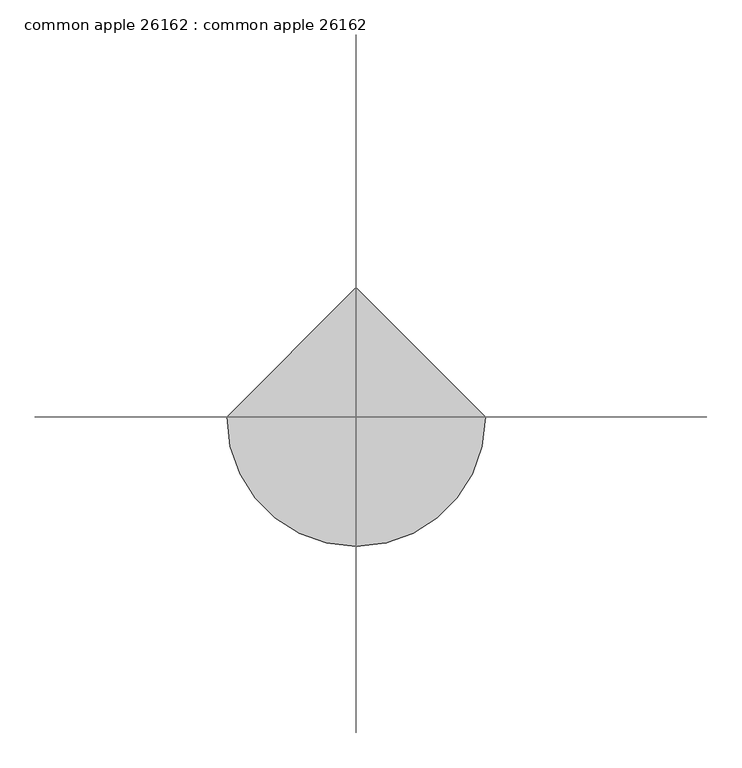
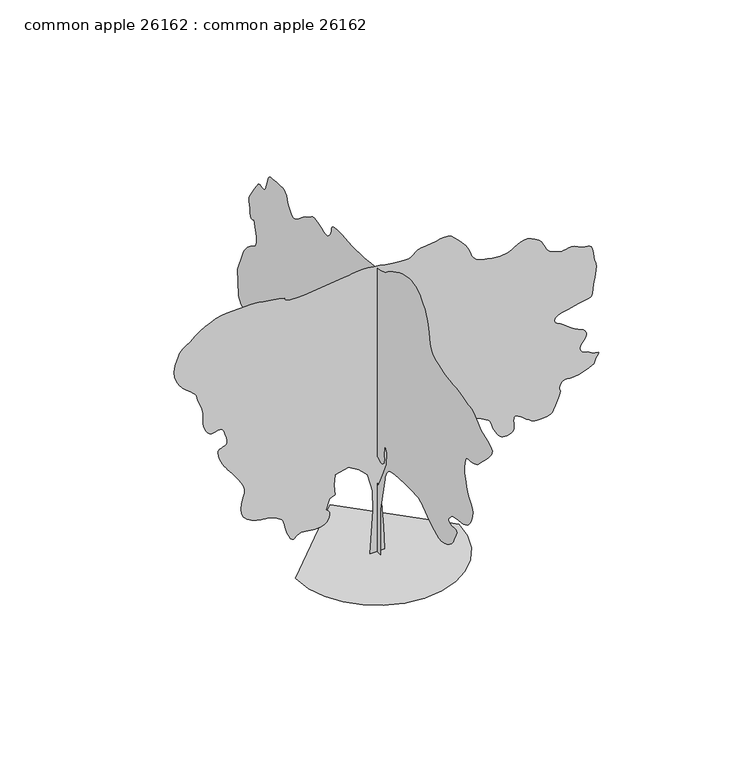
"""IFC4 building model written with IfcOpenShell, lengths in millimetres: proxy geometry, common apple 26162 : common apple 26162."""

import ifcopenshell
import ifcopenshell.guid

model = None  # the IFC model being written
_history = None  # IfcOwnerHistory: only IFC2X3 demands one
_inside = {}  # id of a spatial element -> (the spatial element, [elements in it])
_under = {}  # id of a project, library or spatial element -> (it, [spatial elements below it])
_declared = {}  # id of a project -> (the project, [libraries it declares])
_typed = {}  # id of a type object -> (the type object, [elements of that type])
_made_of = {}  # id of a material, layer set ... -> (it, [elements and type objects made of it])


def new_model(schema):
    """Start an empty IFC model of exactly this schema.

    Asked for "IFC4X3", IfcOpenShell would pick the latest addendum, in which some entities
    have other attributes; the version numbers below select the first issue.
    IFC2X3 requires an IfcOwnerHistory on every rooted entity: one is made here for all.
    """
    global model, _history
    if schema == "IFC4X3":
        model = ifcopenshell.file(schema_version=(4, 3, 0, 0))
    else:
        model = ifcopenshell.file(schema=schema)
    _inside.clear()
    _under.clear()
    _declared.clear()
    _typed.clear()
    _made_of.clear()
    _history = None
    if model.schema == "IFC2X3":
        org = make("IfcOrganization", Name="unknown")
        user = make(
            "IfcPersonAndOrganization",
            ThePerson=make("IfcPerson", FamilyName="unknown"),
            TheOrganization=org,
        )
        app = make(
            "IfcApplication",
            ApplicationDeveloper=org,
            Version="unknown",
            ApplicationFullName="unknown",
            ApplicationIdentifier="unknown",
        )
        _history = make(
            "IfcOwnerHistory",
            OwningUser=user,
            OwningApplication=app,
            ChangeAction="ADDED",
            CreationDate=0,
        )
    return model


def make(cls, **values):
    """One entity of the class cls with the attributes given. An attribute that is None is left unset."""
    return model.create_entity(
        cls, **{name: value for name, value in values.items() if value is not None}
    )


def rooted(cls, **values):
    """An entity with a GlobalId (a new one), such as an element, a storey or a relation."""
    return make(cls, GlobalId=ifcopenshell.guid.new(), OwnerHistory=_history, **values)


def si_unit(unit_type, name, prefix=None):
    """IfcSIUnit, for example si_unit("LENGTHUNIT", "METRE", prefix="MILLI")."""
    return make("IfcSIUnit", UnitType=unit_type, Prefix=prefix, Name=name)


def assignment(units):
    """IfcUnitAssignment: the units of a project."""
    return None if units is None else make("IfcUnitAssignment", Units=units)


def point(xyz):
    """IfcCartesianPoint."""
    return None if xyz is None else make("IfcCartesianPoint", Coordinates=xyz)


def direction(xyz):
    """IfcDirection."""
    return None if xyz is None else make("IfcDirection", DirectionRatios=xyz)


def frame(location, z_axis=None, x_axis=None):
    """IfcAxis2Placement3D, a coordinate frame: its origin and axes. An axis left out is left unset."""
    return make(
        "IfcAxis2Placement3D",
        Location=point(location),
        Axis=direction(z_axis),
        RefDirection=direction(x_axis),
    )


def origin():
    """The frame at (0, 0, 0) with its axes left unset."""
    return frame((0.0, 0.0, 0.0))


def place(relative_to, where):
    """IfcLocalPlacement: puts the frame where relative to a parent placement (None: the world)."""
    return make(
        "IfcLocalPlacement", PlacementRelTo=relative_to, RelativePlacement=where
    )


def context(
    kind, dimensions, precision=None, world=None, true_north=None, identifier=None
):
    """IfcGeometricRepresentationContext, for example the 3D "Model" context."""
    return make(
        "IfcGeometricRepresentationContext",
        ContextIdentifier=identifier,
        ContextType=kind,
        CoordinateSpaceDimension=dimensions,
        Precision=precision,
        WorldCoordinateSystem=world,
        TrueNorth=true_north,
    )


def project(units=None, contexts=None):
    """IfcProject with its units and contexts."""
    return rooted(
        "IfcProject",
        Name="project",
        RepresentationContexts=contexts,
        UnitsInContext=assignment(units),
    )


def spatial(cls, under=None, at=None, **own):
    """A site, building, storey or space (cls), placed at a placement, below another one or the project."""
    s = rooted(cls, ObjectPlacement=at, **own)
    if under is not None:
        _under.setdefault(under.id(), (under, []))[1].append(s)
    return s


def point_list(points):
    """IfcCartesianPointList2D or 3D."""
    cls = (
        "IfcCartesianPointList2D" if len(points[0]) == 2 else "IfcCartesianPointList3D"
    )
    return make(cls, CoordList=points)


def triangles(points, corners, closed=None, point_numbers=None):
    """IfcTriangulatedFaceSet: each triangle names its three corners, points numbered from 1."""
    return make(
        "IfcTriangulatedFaceSet",
        Coordinates=point_list(points),
        Closed=closed,
        CoordIndex=corners,
        PnIndex=point_numbers,
    )


def shape(context_of_items, identifier, shape_type, items):
    """IfcShapeRepresentation: the items that make up one representation, for example the "Body"."""
    return make(
        "IfcShapeRepresentation",
        ContextOfItems=context_of_items,
        RepresentationIdentifier=identifier,
        RepresentationType=shape_type,
        Items=items,
    )


def source(mapping_origin, context_of_items, identifier, shape_type, items):
    """IfcRepresentationMap: a shape defined once, which mapped items show again and again."""
    return make(
        "IfcRepresentationMap",
        MappingOrigin=mapping_origin,
        MappedRepresentation=shape(context_of_items, identifier, shape_type, items),
    )


def transform(
    local_origin,
    x_axis=None,
    y_axis=None,
    z_axis=None,
    scale=None,
    scale2=None,
    scale3=None,
    uniform=True,
):
    """IfcCartesianTransformationOperator3D, or its non-uniform kind. x_axis, y_axis, z_axis: its Axis1, 2, 3."""
    if uniform:
        return make(
            "IfcCartesianTransformationOperator3D",
            Axis1=direction(x_axis),
            Axis2=direction(y_axis),
            LocalOrigin=point(local_origin),
            Scale=scale,
            Axis3=direction(z_axis),
        )
    return make(
        "IfcCartesianTransformationOperator3DnonUniform",
        Axis1=direction(x_axis),
        Axis2=direction(y_axis),
        LocalOrigin=point(local_origin),
        Scale=scale,
        Axis3=direction(z_axis),
        Scale2=scale2,
        Scale3=scale3,
    )


def mapped(mapping_source, mapping_target):
    """IfcMappedItem: shows the shape of a source again, moved by a transform."""
    return make(
        "IfcMappedItem", MappingSource=mapping_source, MappingTarget=mapping_target
    )


def made_of(thing, what):
    """Note that an element or type object is made of a material, layer set ...; save() writes the relation."""
    if what is not None:
        _made_of.setdefault(what.id(), (what, []))[1].append(thing)
    return thing


def element(
    cls,
    number,
    at=None,
    inside=None,
    cuts=None,
    type_object=None,
    material=None,
    context=None,
    identifier="Body",
    shape_type=None,
    held_by="IfcProductDefinitionShape",
    body=None,
    shapes=None,
    **own,
):
    """One element of the class cls, such as IfcWall. Its Tag is "e" and its number.

    at: its placement. inside: the storey or other place that contains it. cuts: it is an
    opening in that element (IfcRelVoidsElement). A single representation is given by context,
    identifier, shape_type and body (its items); several are given by shapes. held_by: the class
    of the entity that holds the representations. save() writes the other relations.
    """
    e = rooted(cls, Tag="e%d" % number, ObjectPlacement=at, **own)
    if body is not None:
        shapes = [shape(context, identifier, shape_type, body)]
    if shapes is not None:
        e.Representation = make(held_by, Representations=shapes)
    if inside is not None:
        _inside.setdefault(inside.id(), (inside, []))[1].append(e)
    if cuts is not None:
        rooted(
            "IfcRelVoidsElement", RelatingBuildingElement=cuts, RelatedOpeningElement=e
        )
    if type_object is not None:
        _typed.setdefault(type_object.id(), (type_object, []))[1].append(e)
    return made_of(e, material)


def aggregate(whole, parts):
    """IfcRelAggregates: a whole, such as a stair, and the parts it consists of."""
    return rooted("IfcRelAggregates", RelatingObject=whole, RelatedObjects=parts)


def save(model, path):
    """Write the relations noted so far, then the file.

    IfcRelAggregates (storeys below a building ...), IfcRelContainedInSpatialStructure (elements
    in a storey), IfcRelDefinesByType, IfcRelAssociatesMaterial and IfcRelDeclares: one each for
    every whole, place, type object, material and project.
    """
    for whole, parts in _under.values():
        aggregate(whole, parts)
    for where, things in _inside.values():
        rooted(
            "IfcRelContainedInSpatialStructure",
            RelatedElements=things,
            RelatingStructure=where,
        )
    for kind, things in _typed.values():
        rooted("IfcRelDefinesByType", RelatedObjects=things, RelatingType=kind)
    for what, things in _made_of.values():
        rooted("IfcRelAssociatesMaterial", RelatedObjects=things, RelatingMaterial=what)
    for by, libraries in _declared.values():
        rooted("IfcRelDeclares", RelatingContext=by, RelatedDefinitions=libraries)
    model.write(path)


def common_apple_26162_common_apple_26162_2cf08d23(model_context):
    return source(origin(), model_context, "Body", "Tessellation", [
        triangles([(-6.61e-05, -106.7031981, 0.0075972), (-6.25e-05, 141.1357166, 0.0075898), (-4.92e-05, 101.4814601, 465.9455781), (-3.19e-05, 131.2220957, 1031.0173004), (-1.83e-05, 230.3576144, 1437.4734501), (-8.7e-06, 398.8869896, 1675.3980263), (-1.1e-06, 587.2459139, 1834.016106), (2.7e-06, 765.6887283, 1873.6680462), (3.6e-06, 963.961219, 1804.2751888), (1.5e-06, 1023.4430534, 1705.1389435), (-4.1e-06, 904.4794573, 1576.2617809), (-8.5e-06, 944.1340136, 1407.7326782), (-1.46e-05, 1172.144878, 1090.4990622), (-1.49e-05, 1568.687534, 882.3128597), (-8.7e-06, 2143.6727863, 803.006436), (7.7e-06, 2490.6473923, 1179.7191977), (2.57e-05, 2847.5453751, 1606.0026981), (3.25e-05, 3402.6882339, 1556.4345028), (3.9e-05, 3600.9610153, 1675.3980263), (4.6e-05, 3591.0549339, 1913.3226025), (4.57e-05, 3412.6196045, 1992.6315697), (5.03e-05, 3283.7399712, 2210.7288677), (5.51e-05, 3591.0549339, 2220.6425068), (6.07e-05, 4205.6845688, 2101.6814541), (6.29e-05, 4275.3567696, 2137.8384041), (6.49e-05, 4342.3114037, 2174.2544952), (6.7e-05, 4403.9061905, 2211.1911942), (6.89e-05, 4457.4241447, 2248.9101128), (7.07e-05, 4500.1976967, 2287.6680668), (7.23e-05, 4529.5348595, 2327.7263775), (7.37e-05, 4542.7427742, 2369.3469475), (8.93e-05, 4572.4863075, 2874.9268433), (9.94e-05, 4403.9570595, 3301.215358), (0.0001002, 4386.5834106, 3334.8449913), (0.000101, 4360.9041641, 3374.6975006), (0.0001018, 4328.265168, 3418.5378479), (0.0001026, 4290.0887192, 3464.105706), (0.0001033, 4247.7471176, 3509.1651649), (0.0001039, 4202.636499, 3551.4561882), (0.0001043, 4156.1291634, 3588.718158), (0.0001045, 4111.323468, 3617.9027138), (0.0001046, 4070.8611122, 3640.1530998), (0.0001046, 4035.4281006, 3659.4571541), (0.0001048, 4005.7101471, 3679.8024239), (0.0001052, 3982.4182549, 3705.2026176), (0.000106, 3966.2384285, 3739.5941231), (0.0001073, 3957.8566727, 3786.9906487), (0.0001089, 3956.7898773, 3842.7945099), (0.0001107, 3961.4378494, 3899.6395866), (0.0001126, 3970.8614021, 3957.3738533), (0.0001145, 3984.0948967, 4015.7685448), (0.0001165, 4000.1982742, 4074.6966339), (0.0001185, 4018.2070587, 4133.9802246), (0.0001206, 4037.1553207, 4193.4417114), (0.0001203, 4062.5299347, 4172.9947037), (0.0001202, 4087.2188347, 4157.4244331), (0.0001204, 4110.5107269, 4151.5570587), (0.000121, 4131.7196068, 4160.2693176), (0.0001221, 4150.160051, 4188.3870781), (0.0001239, 4165.1460548, 4240.787368), (0.0001265, 4175.9410355, 4322.3213448), (0.000129, 4186.6092796, 4402.5600517), (0.0001308, 4198.1408432, 4455.5698975), (0.000132, 4205.3543564, 4492.9588943), (0.000133, 4202.9922913, 4526.3597626), (0.0001339, 4185.923275, 4567.406385), (0.0001352, 4148.8900703, 4627.7059021), (0.000137, 4086.736306, 4718.8666168), (0.0001389, 4019.8834099, 4816.9867905), (0.0001404, 3969.4896835, 4892.043837), (0.0001414, 3931.4405525, 4946.4759796), (0.0001421, 3901.5194138, 4982.6714447), (0.0001423, 3875.5858223, 5003.1184525), (0.0001421, 3849.5002052, 5010.2046478), (0.0001416, 3819.0709579, 5006.343837), (0.0001408, 3787.3208611, 4996.7176804), (0.0001401, 3759.4062859, 4987.6240494), (0.0001396, 3734.2601463, 4983.2045517), (0.0001394, 3710.841227, 4987.6240494), (0.0001396, 3688.1338921, 5005.0485672), (0.0001402, 3665.0704742, 5039.6435486), (0.0001416, 3640.6103394, 5095.574437), (0.0001432, 3619.2235634, 5160.9030075), (0.0001447, 3603.043737, 5219.9581238), (0.000146, 3587.5496246, 5271.4183548), (0.000147, 3568.2455704, 5313.8366959), (0.0001475, 3540.6103386, 5345.8661362), (0.0001475, 3500.1482735, 5366.109668), (0.0001469, 3442.3378487, 5373.1458664), (0.0001459, 3372.4368828, 5376.2445145), (0.0001451, 3300.6055115, 5383.3312912), (0.0001442, 3229.8412262, 5391.1034912), (0.0001434, 3163.0391991, 5396.2851517), (0.0001425, 3103.1713417, 5395.5485687), (0.0001414, 3053.2095657, 5385.642778), (0.0001402, 3016.0746231, 5363.2394943), (0.0001391, 2991.8429626, 5337.2044556), (0.0001382, 2976.4758774, 5316.3510773), (0.0001375, 2966.6462448, 5297.4283951), (0.0001368, 2959.0769394, 5277.1081238), (0.0001359, 2950.4664185, 5252.1148819), (0.0001348, 2937.5122673, 5219.1198029), (0.0001331, 2916.9382324, 5174.873085), (0.0001313, 2890.1666107, 5126.1051315), (0.0001296, 2860.6265533, 5083.2042618), (0.000128, 2827.9619774, 5048.4569641), (0.0001268, 2791.8432518, 5024.124147), (0.0001258, 2751.8890045, 5012.4399765), (0.0001253, 2707.794603, 5015.6909409), (0.0001252, 2659.1789658, 5036.0873703), (0.0001254, 2610.791803, 5068.0662323), (0.0001258, 2565.8846603, 5103.6768494), (0.0001263, 2521.8332794, 5141.7006912), (0.0001267, 2476.0523529, 5180.9436447), (0.0001272, 2425.9356445, 5220.212178), (0.0001274, 2368.8821503, 5258.2360199), (0.0001275, 2302.2908661, 5293.846637), (0.0001276, 2240.2945049, 5328.4671982), (0.0001279, 2193.5584042, 5362.0459625), (0.0001282, 2154.2798424, 5391.129071), (0.0001282, 2114.6558075, 5412.2365036), (0.0001278, 2066.8783459, 5421.8882401), (0.0001267, 2003.1496777, 5416.6304214), (0.0001247, 1915.6618492, 5392.9830276), (0.0001224, 1826.1497257, 5361.2837997), (0.0001207, 1757.9710384, 5335.9853439), (0.0001194, 1705.7434124, 5319.8816757), (0.0001187, 1664.0950825, 5315.7418121), (0.0001184, 1627.6484699, 5326.358606), (0.0001187, 1591.0293388, 5354.4766571), (0.0001195, 1548.8602558, 5402.8893997), (0.0001207, 1514.8419834, 5459.7853455), (0.000122, 1498.8602554, 5510.7630478), (0.0001232, 1489.8128426, 5554.806871), (0.0001241, 1476.6047825, 5590.874437), (0.0001244, 1448.1338459, 5617.9256927), (0.0001241, 1393.3079773, 5634.9182602), (0.0001229, 1301.0220406, 5640.8109238), (0.0001214, 1201.3955635, 5639.6935501), (0.0001202, 1126.7398006, 5636.6454803), (0.0001192, 1069.2519579, 5632.2259827), (0.0001184, 1021.1290958, 5626.9425842), (0.0001175, 974.5682751, 5621.3039749), (0.0001165, 921.7642307, 5615.8426804), (0.0001154, 854.9113346, 5611.0679718), (0.0001143, 784.7082069, 5608.019902), (0.0001133, 723.0014357, 5607.2071609), (0.0001125, 663.7228592, 5608.4768509), (0.0001116, 600.8019178, 5611.6516571), (0.0001107, 528.1680156, 5616.5792633), (0.0001096, 439.7556433, 5623.0567749), (0.0001082, 329.4941322, 5630.9051331), (0.0001067, 206.9466705, 5641.7254028), (0.0001053, 88.3885184, 5656.6861176), (0.0001042, -22.1921751, 5675.1262711), (0.0001034, -120.8075788, 5696.3354416), (0.0001029, -203.4686488, 5719.6276245), (0.0001027, -266.1871316, 5744.3162338), (0.0001028, -304.9729546, 5769.6908478), (0.0001032, -347.9523442, 5804.4381454), (0.0001036, -420.583703, 5853.4089935), (0.0001039, -514.8939712, 5910.1532043), (0.000104, -622.9024584, 5968.31884), (0.0001039, -736.6335978, 6021.4301331), (0.0001035, -848.1092062, 6063.1118912), (0.0001027, -949.3562239, 6086.9371811), (0.0001016, -1039.2697763, 6095.8017563), (0.0001004, -1122.4243664, 6096.0046509), (9.9e-05, -1199.3330441, 6086.1494385), (9.73e-05, -1270.5191059, 6064.8391113), (9.53e-05, -1336.5033051, 6030.7016602), (9.29e-05, -1397.8062492, 5982.3650757), (9.01e-05, -1454.9462208, 5918.407933), (8.77e-05, -1502.3755932, 5861.1056168), (8.62e-05, -1536.9730453, 5825.4944183), (8.5e-05, -1562.8963177, 5799.256485), (8.38e-05, -1584.313615, 5770.0716385), (8.22e-05, -1605.3828232, 5725.6220261), (7.96e-05, -1630.2698215, 5653.5874695), (7.58e-05, -1663.1323505, 5541.6751144), (7.16e-05, -1693.8258259, 5415.6147858), (6.81e-05, -1715.6747829, 5307.5626602), (6.5e-05, -1738.0446384, 5214.9799393), (6.21e-05, -1770.3000824, 5135.1981812), (5.93e-05, -1821.8062408, 5065.6530075), (5.62e-05, -1901.9230076, 5003.7532974), (5.28e-05, -2020.0178341, 4946.8823502), (4.95e-05, -2152.913356, 4902.7117905), (4.69e-05, -2273.494804, 4876.3974083), (4.48e-05, -2385.2295536, 4861.5384315), (4.29e-05, -2491.5921021, 4851.7340881), (4.1e-05, -2596.0345642, 4840.5071571), (3.89e-05, -2702.0542557, 4821.482737), (3.62e-05, -2813.1030006, 4788.2594742), (3.39e-05, -2912.3155495, 4758.5159409), (3.24e-05, -2986.585144, 4746.9843773), (3.14e-05, -3044.8780975, 4742.742485), (3.04e-05, -3096.2371719, 4734.8432579), (2.89e-05, -3149.6786774, 4712.3896866), (2.66e-05, -3214.2200867, 4664.4344742), (2.28e-05, -3298.878582, 4580.0809021), (1.85e-05, -3408.6320572, 4492.8062874), (1.5e-05, -3530.0185432, 4434.3354378), (1.2e-05, -3644.3188339, 4390.95233), (9.4e-06, -3732.7616913, 4348.9659393), (7.2e-06, -3776.6273277, 4294.6608238), (5.1e-06, -3757.196537, 4214.3459587), (3e-06, -3655.7486595, 4094.3056114), (1.1e-06, -3529.027906, 3968.7786804), (-3e-07, -3439.3912262, 3876.7287758), (-1.3e-06, -3376.6531952, 3811.5525215), (-1.9e-06, -3330.5522301, 3766.670668), (-2.3e-06, -3290.852037, 3735.479258), (-2.3e-06, -3247.3671913, 3711.4002045), (-2.2e-06, -3189.8108208, 3687.854258), (-1.7e-06, -3124.3802216, 3671.1919029), (-1e-06, -3064.487075, 3666.3404549), (-2e-07, -3010.8420937, 3664.4356293), (2e-07, -2964.1568619, 3656.6378494), (2e-07, -2925.0662247, 3634.0825401), (-8e-07, -2894.3070557, 3587.9559952), (-2.8e-06, -2872.5897766, 3509.3939301), (-5.1e-06, -2860.8041588, 3423.8465355), (-7.1e-06, -2858.3659355, 3357.9081184), (-8.8e-06, -2863.7507813, 3304.4410332), (-1.04e-05, -2875.358503, 3256.3335045), (-1.21e-05, -2891.6653564, 3206.498465), (-1.41e-05, -2911.070858, 3147.8244301), (-1.67e-05, -2932.0768433, 3073.199334), (-1.95e-05, -2961.2613991, 2993.8242371), (-2.22e-05, -3001.7234642, 2923.6186386), (-2.47e-05, -3046.5291595, 2859.6612053), (-2.72e-05, -3088.7187355, 2798.9806068), (-2.95e-05, -3121.3830208, 2738.6555099), (-3.16e-05, -3137.5628471, 2675.7398735), (-3.35e-05, -3130.349334, 2607.2612045), (-3.52e-05, -3109.3942177, 2540.281572), (-3.66e-05, -3087.7280983, 2482.819091), (-3.77e-05, -3063.4964378, 2433.5098915), (-3.85e-05, -3034.7182526, 2390.964814), (-3.91e-05, -2999.5645844, 2353.7970245), (-3.94e-05, -2956.0544495, 2320.6169277), (-3.96e-05, -2902.3333099, 2290.0378349), (-3.93e-05, -2836.3948929, 2266.2507694), (-3.86e-05, -2760.9314758, 2251.4832115), (-3.77e-05, -2680.9721123, 2241.3942924), (-3.68e-05, -2601.4955681, 2231.6559334), (-3.61e-05, -2527.6041481, 2217.9272655), (-3.58e-05, -2464.279525, 2195.8749779), (-3.62e-05, -2416.56049, 2161.1632885), (-3.68e-05, -2383.2356346, 2123.2410393), (-3.73e-05, -2359.9691769, 2093.2995529), (-3.79e-05, -2347.1065899, 2069.598674), (-3.84e-05, -2344.9984337, 2050.4090023), (-3.9e-05, -2353.9875652, 2033.9929985), (-3.98e-05, -2374.4217831, 2018.6158848), (-4.07e-05, -2406.646851, 2002.5452087), (-4.16e-05, -2449.8269188, 1993.9041664), (-4.23e-05, -2498.3841293, 1996.5330757), (-4.28e-05, -2545.5646797, 2002.2862129), (-4.34e-05, -2584.5791588, 2003.0075352), (-4.41e-05, -2608.6837921, 1990.5513187), (-4.52e-05, -2611.0967262, 1956.7642822), (-4.66e-05, -2585.0869766, 1893.4953243), (-4.83e-05, -2549.9080193, 1821.1814243), (-4.96e-05, -2524.6272949, 1762.91376), (-5.07e-05, -2502.1126808, 1714.5318295), (-5.16e-05, -2475.2625755, 1671.8725147), (-5.23e-05, -2436.9668026, 1630.7726978), (-5.27e-05, -2380.1140228, 1587.0720222), (-5.3e-05, -2297.5969666, 1536.6072247), (-5.28e-05, -2203.8378639, 1496.8968578), (-5.19e-05, -2116.842738, 1484.7582092), (-5.03e-05, -2034.8743401, 1494.9892708), (-4.83e-05, -1956.2028339, 1522.3883251), (-4.6e-05, -1879.090971, 1561.7532188), (-4.35e-05, -1801.803828, 1607.8822346), (-4.09e-05, -1722.6115688, 1655.5707481), (-3.83e-05, -1647.9584221, 1703.6352562), (-3.59e-05, -1583.013113, 1752.3931812), (-3.37e-05, -1524.1383636, 1798.8980461), (-3.16e-05, -1467.6919544, 1840.2010483), (-2.97e-05, -1410.0313751, 1873.3506237), (-2.82e-05, -1347.5167316, 1895.4053822), (-2.69e-05, -1276.503479, 1903.4089634), (-2.54e-05, -1177.6846561, 1904.2776604), (-2.33e-05, -1044.3574018, 1905.4916851), (-2.11e-05, -891.7820492, 1904.9710773), (-1.89e-05, -735.2163151, 1900.6352955), (-1.7e-05, -589.9230761, 1890.4040886), (-1.58e-05, -471.1627742, 1872.1948803), (-1.55e-05, -394.1956335, 1843.9297451), (-1.6e-05, -348.7041879, 1805.3140789), (-1.68e-05, -313.0958962, 1758.377409), (-1.8e-05, -285.7248199, 1704.5039532), (-1.95e-05, -264.9450744, 1645.0805454), (-2.11e-05, -249.1058704, 1581.494165), (-2.29e-05, -236.5620685, 1515.1341167), (-2.48e-05, -225.6659676, 1447.3870892), (-3.91e-05, -116.6168281, 912.0537769), (-2.05e-05, -27.3946828, 1318.5099266), (-1.32e-05, -176.0980811, 1635.74347), (-6.6e-06, -304.975498, 1923.2362415), (2e-07, -324.8002327, 2161.1632885), (4.8e-06, -255.4073572, 2280.1241959), (-4e-07, -225.6657133, 2091.767815), (-1.7e-06, -231.7353101, 2049.4539734), (-3e-06, -235.984215, 2008.1814926), (-4.2e-06, -236.5910275, 1968.9892628), (-5.2e-06, -231.7353101, 1932.9186447), (-6e-06, -219.5961346, 1901.0111446), (-6.5e-06, -198.3530817, 1874.3056526), (-6.6e-06, -166.1844602, 1853.8433842), (-6.2e-06, -129.2182845, 1848.5829494), (-5.3e-06, -95.0268123, 1860.3152275), (-4.3e-06, -63.9562343, 1879.3348515), (-3.4e-06, -36.354542, 1895.9235191), (-2.9e-06, -12.5678035, 1900.3761543), (-3.1e-06, 7.0569383, 1882.9772163), (-4.4e-06, 22.1729471, 1834.016106), (-6.1e-06, 32.8958209, 1768.9260384), (-7.8e-06, 39.9768386, 1709.0403042), (-9.4e-06, 44.0233167, 1653.4904972), (-1.1e-05, 45.6418044, 1601.4077751), (-1.24e-05, 45.4396183, 1551.9260571), (-1.39e-05, 44.0233167, 1504.1789715), (-1.53e-05, 41.9999482, 1457.3007282), (139.590126, 0.0003305, 0.0), (-135.4471285, 0.0003387, 0.0), (-74.3278259, 0.000241, 845.4879272), (-84.5142454, 0.0002472, 1242.76455), (-186.3807747, 0.0002013, 1599.294532), (-339.1791879, 0.0002082, 1752.0933449), (-542.9102117, 0.000216, 1874.3335579), (-797.5758808, 0.0002227, 1813.2134514), (-817.9492012, 0.0002203, 1609.4824276), (-797.5758808, 0.0002168, 1415.9368286), (-899.4426281, 0.0002191, 1365.0021469), (-970.7481594, 0.0002183, 1171.4565479), (-951.3247084, 0.0002718, 1158.1240768), (-933.2373676, 0.000271, 1143.3616058), (-917.8246456, 0.0002703, 1125.7517796), (-906.4200365, 0.0002696, 1103.8645981), (-900.3621214, 0.000269, 1076.2750757), (-900.9870106, 0.0002686, 1041.555756), (-909.6280529, 0.0002682, 998.2868128), (-928.5764603, 0.0002681, 955.1042742), (-957.6798437, 0.0002684, 921.0098436), (-994.6267164, 0.0002692, 895.1144766), (-1037.0955631, 0.0002701, 876.5217161), (-1082.7698101, 0.0002713, 864.3449158), (-1129.3382612, 0.0002726, 857.6926329), (-1174.4791832, 0.0002739, 855.6733521), (-1218.6700905, 0.0002753, 858.4063974), (-1263.5747623, 0.0002767, 865.0586803), (-1308.6573303, 0.0002782, 873.3161705), (-1353.3816353, 0.0002796, 880.857498), (-1397.217041, 0.000281, 885.3710306), (-1439.6273884, 0.0002823, 884.5404854), (-1480.0769543, 0.0002833, 876.0466724), (-1514.854628, 0.0002841, 857.900905), (-1542.5051205, 0.0002846, 834.4084436), (-1565.8782578, 0.000285, 812.6990856), (-1587.8238659, 0.0002854, 799.9000122), (-1611.1970032, 0.0002862, 803.1359339), (-1638.8473503, 0.0002874, 829.5392641), (-1673.6225533, 0.000235, 886.2346407), (-1706.6171963, 0.0002371, 959.4984827), (-1729.2790398, 0.0002388, 1029.5593225), (-1744.988982, 0.0002402, 1094.4487484), (-1757.1353336, 0.0002415, 1152.2135365), (-1769.1037891, 0.0002426, 1200.8900711), (-1784.2803337, 0.0002436, 1238.5177162), (-1806.0481911, 0.0002446, 1263.1378704), (-1833.1626698, 0.0002457, 1282.7670502), (-1863.3073414, 0.0002469, 1305.4288937), (-1898.2629112, 0.0002483, 1329.1576778), (-1939.8122646, 0.0002499, 1351.9948013), (-1989.7334908, 0.0002517, 1371.9820988), (-2049.8147072, 0.0002537, 1387.1586433), (-2121.8338577, 0.000256, 1395.5635082), (-2205.4938675, 0.0002044, 1404.6210949), (-2294.67854, 0.0002073, 1424.3695988), (-2382.4381542, 0.0002104, 1456.7724174), (-2461.8232796, 0.0002135, 1503.7853909), (-2525.8821602, 0.0002163, 1567.3691551), (-2567.6627495, 0.0002188, 1649.4849277), (-2580.2355286, 0.0002207, 1752.0933449), (-2568.9835991, 0.0002218, 1851.4048702), (-2548.8159348, 0.0002224, 1927.9097935), (-2527.0379036, 0.0002227, 1989.979842), (-2510.9723145, 0.0001688, 2045.9893593), (-2507.9117455, 0.0001695, 2104.3180664), (-2525.1659248, 0.0001711, 2173.3375454), (-2570.0503944, 0.0001737, 2261.4222851), (-2629.7912247, 0.0001769, 2355.7756828), (-2686.3316689, 0.0001798, 2438.7243988), (-2738.9604332, 0.0001825, 2511.3356644), (-2786.9665146, 0.0001849, 2574.6730774), (-2829.6130394, 0.0001327, 2629.841803), (-2866.1890045, 0.0001345, 2677.8478844), (-2896.008696, 0.000136, 2719.8086952), (-2924.6092758, 0.0001376, 2767.4084061), (-2955.1652596, 0.0001394, 2827.2762634), (-2983.4100471, 0.0001412, 2893.0114952), (-3005.0764572, 0.0001428, 2958.2389091), (-3015.8461487, 0.000144, 3016.5062828), (-3011.4772293, 0.0001446, 3061.4137161), (-2987.7028084, 0.0001442, 3086.5342758), (-2951.4823448, 0.0001433, 3098.8532913), (-2915.109565, 0.0001425, 3111.5533882), (-2882.1147766, 0.0001417, 3127.4282913), (-2856.0800285, 0.0001413, 3149.3740448), (-2840.5350471, 0.0001413, 3180.2349518), (-2839.0871704, 0.0001418, 3222.8561874), (-2855.2669968, 0.0001432, 3280.0823456), (-2877.0348541, 9.05e-05, 3338.9342766), (-2892.2240433, 9.16e-05, 3385.5177704), (-2904.1875572, 9.25e-05, 3421.2048363), (-2916.3286766, 9.32e-05, 3447.4686401), (-2932.0259743, 9.4e-05, 3465.705899), (-2954.70802, 9.48e-05, 3477.3389099), (-2987.7028084, 9.59e-05, 3483.8161308), (-3026.4123642, 9.7e-05, 3481.8857254), (-3064.2583099, 9.8e-05, 3472.1066711), (-3101.5455688, 9.9e-05, 3461.6419029), (-3138.6805115, 0.0001, 3457.552327), (-3175.9930595, 0.0001013, 3467.026458), (-3213.8137161, 0.0001029, 3497.1763618), (-3252.5488518, 0.0001049, 3555.1138138), (-3281.1747208, 0.0001068, 3626.7419998), (-3293.239682, 0.0001082, 3695.3474052), (-3295.8558014, 0.0001093, 3764.1307068), (-3296.1351448, 0.0001104, 3836.3175797), (-3301.2406471, 5.74e-05, 3915.0575409), (-3318.2840836, 5.93e-05, 4003.6274254), (-3354.4028091, 6.19e-05, 4105.2020393), (-3391.2836975, 6.43e-05, 4197.0231789), (-3411.2481766, 6.59e-05, 4259.8120789), (-3422.2972115, 6.68e-05, 4301.925206), (-3432.4570564, 6.76e-05, 4331.7448975), (-3449.7545471, 6.85e-05, 4357.6276199), (-3482.1650688, 6.99e-05, 4387.9804184), (-3537.7657448, 7.22e-05, 4431.1606316), (-3609.6985634, 2.09e-05, 4488.5646858), (-3681.631382, 2.41e-05, 4556.1285851), (-3747.3157448, 2.72e-05, 4634.0305161), (-3800.5287758, 3.01e-05, 4722.4480843), (-3835.047599, 3.26e-05, 4821.5588951), (-3844.6231773, 3.45e-05, 4931.5152649), (-3822.9823471, 3.57e-05, 5052.5468307), (-3789.555899, -1.8e-05, 5157.9310959), (-3763.7749146, -1.77e-05, 5228.187854), (-3739.5941231, -1.77e-05, 5274.3902664), (-3710.9682541, -1.81e-05, 5307.5882401), (-3671.8270386, -1.88e-05, 5338.8555176), (-3616.1246246, -1.98e-05, 5379.1652664), (-3537.7657448, -2.13e-05, 5439.6429703), (-3445.4364967, -2.3e-05, 5511.6775269), (-3351.6849518, -2.48e-05, 5578.225209), (-3256.3079247, -2.67e-05, 5637.4326416), (-3159.1783882, -2.89e-05, 5687.5726044), (-3060.0675774, -3.12e-05, 5726.8155579), (-2958.8228851, -3.39e-05, 5753.4348633), (-2855.2669968, -3.68e-05, 5765.6015625), (-2376.4970924, -5.09e-05, 5775.7869873), (-2309.7356152, -5.29e-05, 5773.1197083), (-2232.8167637, -5.53e-05, 5765.6521408), (-2147.4320045, -3.8e-06, 5754.1458664), (-2055.2781818, -6.7e-06, 5739.4392059), (-1958.0469074, -9.9e-06, 5722.3449005), (-1857.4273224, -1.32e-05, 5703.6251129), (-1755.1159801, -1.65e-05, 5684.1181641), (-1751.9080364, -1.69e-05, 5664.6617935), (-1742.5530842, -1.75e-05, 5646.3739563), (-1720.9022255, -1.83e-05, 5630.3970245), (-1680.8107773, -1.97e-05, 5617.9001129), (-1616.1270802, -2.18e-05, 5610.0261749), (-1520.7042709, -2.46e-05, 5607.9437439), (-1388.3981026, -2.85e-05, 5612.8201904), (-614.2181774, -5.02e-05, 5704.4890137), (-538.3076946, -5.24e-05, 5711.4996323), (-472.1990845, 1e-07, 5721.8879517), (-409.4762778, -1.6e-06, 5732.8355392), (-343.7232419, -3.5e-06, 5741.4460602), (-268.5264692, -5.7e-06, 5744.8749207), (-177.4707081, -8.5e-06, 5740.3031067), (-64.1414019, -1.21e-05, 5724.8598633), (54.7118994, -1.59e-05, 5704.3111176), (159.4882483, -1.93e-05, 5686.4296509), (252.3260954, -2.23e-05, 5671.4183578), (335.3640864, -2.49e-05, 5659.4039749), (410.7386644, -2.73e-05, 5650.6155579), (480.5886887, -2.95e-05, 5645.205423), (547.0529457, -3.15e-05, 5643.3764648), (603.2428662, -3.3e-05, 5651.8346695), (646.0698669, -3.4e-05, 5673.6531052), (683.3697704, -3.47e-05, 5703.4983765), (722.9887184, -3.54e-05, 5736.0359253), (772.7625698, -3.64e-05, 5765.8806152), (840.5349592, -3.81e-05, 5787.6996323), (934.1441437, -4.07e-05, 5796.1828354), (1035.6832947, -4.37e-05, 5802.989978), (1124.0372766, -4.61e-05, 5818.3826431), (1202.2337391, -4.82e-05, 5834.6642075), (1273.3004768, -5.01e-05, 5844.1636276), (1340.2726971, -5.22e-05, 5839.2360214), (1406.173035, -5.46e-05, 5812.2103455), (1474.0342999, -3.2e-06, 5755.4161377), (1539.0152172, -6.2e-06, 5686.9627579), (1594.7301304, -8.7e-06, 5628.1366974), (1641.8903332, -1.09e-05, 5576.0666199), (1681.2120609, -1.28e-05, 5527.9335114), (1713.4041367, -1.44e-05, 5480.8671982), (1739.182505, -1.59e-05, 5431.9975067), (1759.2587505, -1.73e-05, 5378.5304214), (1777.3156425, -1.87e-05, 5324.8604416), (1798.9361252, -2e-05, 5277.2604401), (1827.6839344, -2.15e-05, 5235.5281036), (1867.1225155, 3.1e-05, 5199.4855362), (1920.8180752, 2.9e-05, 5169.0060013), (1992.3318787, 2.65e-05, 5143.8342819), (2085.229842, 2.34e-05, 5123.844223), (2181.6306438, 2.03e-05, 5109.4171967), (2262.7075264, 1.78e-05, 5100.6799393), (2330.5991673, 1.57e-05, 5097.123761), (2387.4419186, 1.4e-05, 5098.1905563), (2435.3767834, 1.27e-05, 5103.3722168), (2476.5374977, 1.16e-05, 5112.0844757), (2513.0678261, 1.07e-05, 5123.844223), (2552.2195061, 9.8e-06, 5144.4947067), (2599.1840813, 8.9e-06, 5175.4829315), (2653.1336952, 7.8e-06, 5209.6459625), (2713.1032906, 6.4e-06, 5239.9226028), (2778.2795448, 4.8e-06, 5259.1249191), (2847.697982, 2.7e-06, 5260.1661346), (2920.5196999, 2e-07, 5235.9094757), (2984.2992371, -2.2e-06, 5202.1528152), (3030.2478859, -4e-06, 5176.5747253), (3062.9883293, -5.3e-06, 5154.908606), (3087.1947006, -6.3e-06, 5132.9122742), (3107.4893921, -7.3e-06, 5106.2679703), (3128.4697975, -8.5e-06, 5070.73293), (3154.8094688, -1e-05, 5021.9905563), (3182.8510712, 4.27e-05, 4971.0890121), (3208.2256851, 4.13e-05, 4930.3473129), (3234.4639091, 4e-05, 4897.4289734), (3265.1724998, 3.87e-05, 4870.0475052), (3303.9076355, 3.72e-05, 4845.8667137), (3354.2252037, 3.53e-05, 4822.6004013), (3419.6808014, 3.3e-05, 4797.8859215), (3486.0258797, 3.08e-05, 4782.8237595), (3540.0769409, 2.92e-05, 4784.7032959), (3586.9909378, 2.8e-05, 4795.4729874), (3631.9489494, 2.68e-05, 4807.1571579), (3680.1326363, 2.55e-05, 4811.7036827), (3736.6730804, 2.36e-05, 4801.0863075), (3806.7519424, 2.1e-05, 4767.3299377), (3879.2181587, 1.84e-05, 4732.9890106), (3939.9240463, 1.63e-05, 4718.4346664), (3989.5811897, 1.48e-05, 4712.2626595), (4028.9003014, 1.35e-05, 4703.0678719), (4058.6185455, 1.22e-05, 4679.4204781), (4079.3957657, 6.51e-05, 4629.9412308), (4091.9941246, 6.34e-05, 4543.2253029), (4103.8306114, 6.18e-05, 4454.6301292), (4119.4261711, 6.04e-05, 4397.0481789), (4135.0217308, 5.94e-05, 4355.3161331), (4146.8835068, 5.84e-05, 4314.2950905), (4151.2268463, 5.74e-05, 4258.8467308), (4144.3688347, 5.64e-05, 4173.8330246), (4122.550399, 5.51e-05, 4044.0642014), (4100.096537, 0.000108, 3908.7329269), (4088.8698967, 0.0001069, 3812.0603394), (4081.3767494, 0.0001061, 3746.5791618), (4070.1501091, 0.0001058, 3704.7962471), (4047.6965378, 0.0001061, 3679.2184479), (4006.548468, 0.0001071, 3662.4034859), (3939.1874634, 0.0001089, 3646.8079262), (3844.4708611, 0.0001114, 3628.5706673), (3734.0822502, 0.0001144, 3608.1998177), (3619.7822502, 0.0001175, 3584.781189), (3513.3053192, 0.0001202, 3557.4761696), (3426.4373657, 0.0001224, 3525.3449913), (3370.9384277, 0.0001234, 3487.4990456), (3358.5429634, 0.0001231, 3443.0744316), (3371.5224037, 0.0001222, 3405.6092766), (3386.2799332, 0.0001214, 3384.1972115), (3405.8633308, 0.0001207, 3371.1669022), (3433.2700882, 0.0001197, 3358.8478867), (3471.5476936, 0.0001182, 3339.5694122), (3523.7447983, 0.0001162, 3305.6857246), (3592.8327324, 0.0001133, 3249.5260712), (3669.2870773, 0.0001101, 3189.9884262), (3740.381575, 0.0001074, 3147.3671906), (3804.5419029, 0.000105, 3116.150782), (3860.1425789, 0.0001572, 3090.8014572), (3905.55783, 0.0001555, 3065.8332138), (3939.2383324, 0.000154, 3035.6833099), (3959.558313, 0.0001528, 2994.8654526), (3960.2948959, 0.0001521, 2946.884951), (3941.8038734, 0.0001519, 2899.2852402), (3912.2635254, 0.0001521, 2852.3968231), (3879.8530037, 0.0001524, 2806.5752014), (3852.8020386, 0.0001525, 2762.1758766), (3839.2892006, 0.0001523, 2719.554641), (3847.5189308, 0.0001514, 2679.0672867), (3870.582058, 0.0001503, 2647.1645828), (3896.1598572, 0.0001492, 2627.2256836), (3924.2270393, 0.0001482, 2614.9319572), (3954.7830231, 0.0001472, 2606.0168037), (3987.8286804, 0.000146, 2596.2121696), (4023.3887192, 0.0001447, 2581.2517456), (4061.4378502, 0.0001432, 2556.842189), (4100.7569618, 0.0001417, 2534.5891869), (4137.7648773, 0.0001405, 2524.8203064), (4168.8798386, 0.0001395, 2521.2847664), (4190.5462486, 0.0001388, 2517.7515518), (4199.2329277, 0.0001384, 2507.9803459), (4191.3334099, 0.0001926, 2485.7375175), (4163.2918076, 0.0001928, 2444.7824593), (4135.3263634, 0.0001929, 2399.7888393), (4122.8550316, 0.0001928, 2366.7332989), (4115.1842789, 0.0001927, 2341.3408081), (4101.6461517, 0.0001927, 2319.3343025), (4071.521537, 0.0001933, 2296.4387524), (4014.1430626, 0.0001946, 2268.3717155), (3918.8166138, 0.0001969, 2230.8633945), (3811.1205711, 0.0001996, 2200.6297749), (3722.1443161, 0.0002021, 2191.0666958), (3649.3987564, 0.0002043, 2192.9081532), (3590.3436401, 0.0002062, 2196.8884335), (3542.540744, 0.0002075, 2193.7413872), (3503.4501068, 0.0002084, 2174.1985394), (3470.6079254, 0.0002087, 2128.9966473), (3451.2532928, 0.0002086, 2081.7474964), (3449.1702805, 0.0002083, 2055.3443115), (3456.7142967, 0.0002078, 2039.4564732), (3466.2137169, 0.0002073, 2023.7466763), (3470.0236588, 0.0002068, 1997.8792145), (3460.4480804, 0.0002064, 1951.5191082), (3429.8662262, 0.0002061, 1874.3335579), (3393.2393921, 0.0002059, 1787.376511), (3366.4171921, 0.0002057, 1717.5239433), (3342.9982727, 0.0002056, 1663.1755165), (3316.5315742, 0.0002058, 1622.7259506), (3280.6157433, 0.0002064, 1594.5725819), (3228.850589, 0.0002077, 1577.1101303), (3154.8094688, 0.0002098, 1568.7357868), (3080.6413216, 0.0002119, 1565.2609989), (3027.8349518, 0.0002135, 1564.6361824), (2989.0998161, 0.0002147, 1568.469088), (2957.146534, 0.0002158, 1578.3572926), (2924.6598541, 0.000217, 1595.9086922), (2884.3248161, 0.0002186, 1622.7259506), (2828.8511673, 0.0002209, 1660.4146385), (2768.830703, 0.0002233, 1702.4363468), (2719.1482704, 0.0002253, 1739.6499184), (2678.9146797, 0.000227, 1769.7336926), (2647.2154518, 0.0002282, 1790.3763279), (2623.1869766, 0.0002291, 1799.2561638), (2605.9403549, 0.0002295, 1794.0567719), (2594.5613983, 0.0002295, 1772.4668106), (2588.1350464, 0.0002293, 1744.7273701), (2585.6459541, 0.000229, 1721.445797), (2586.0014557, 0.0002287, 1700.833683), (2588.1350464, 0.0002283, 1681.1130844), (2591.00522, 0.0002279, 1660.5034412), (2593.494603, 0.0002275, 1637.219252), (2594.5613983, 0.0002271, 1609.4824276), (2593.1135216, 0.0002267, 1579.0989624), (2587.906572, 0.0002264, 1549.7873795), (2577.7211472, 0.0002263, 1522.6143288), (2561.2872665, 0.0002264, 1498.6468964), (2537.3884346, 0.0002268, 1478.9568192), (2504.7494385, 0.0002276, 1464.6108925), (2462.1331444, 0.0002288, 1456.6836147), (2418.7144283, 0.00023, 1454.9893867), (2382.9562912, 0.0002312, 1459.35569), (2352.5447754, 0.0002322, 1470.8491745), (2325.1635979, 0.0002333, 1490.5392517), (2298.4935688, 0.0002346, 1519.4951878), (2270.2207306, 0.000236, 1558.7865395), (2238.0288002, 0.0002377, 1609.4824276), (2208.2396301, 0.0002394, 1664.8392231), (2186.8274197, 0.0001866, 1716.8127949), (2170.9397266, 0.0001878, 1764.5088661), (2157.7241089, 0.0001888, 1807.0362122), (2144.3307404, 0.0001897, 1843.5054977), (2127.9070335, 0.0001907, 1873.0254982), (2105.6033077, 0.0001917, 1894.7068783), (2074.6583942, 0.0001929, 1913.6528149), (2035.1589157, 0.0001944, 1935.2732975), (1988.5319653, 0.0001961, 1959.1214058), (1936.2028919, 0.0001981, 1984.7525448), (1879.5964634, 0.0002001, 2011.717178), (1820.1400635, 0.0002023, 2039.5759426), (1759.2587505, 0.0002046, 2067.8791569), (1412.9141933, 0.0002149, 2067.8791569), (1219.3685944, 0.0002173, 1843.7721966), (1214.8270838, 0.000217, 1813.2134514), (1209.2136909, 0.0002167, 1782.6522354), (1201.4616205, 0.0002165, 1752.0933449), (1190.5040045, 0.0002164, 1721.5345997), (1175.2665625, 0.0002164, 1690.9733837), (1154.6874407, 0.0002165, 1660.4146385), (1127.6898153, 0.0002169, 1629.855748), (1103.6638836, 0.0002172, 1604.0163368), (1088.903956, 0.0002174, 1586.5538853), (1077.7076191, 0.0002175, 1575.8629681), (1064.3726046, 0.0002179, 1570.3384506), (1043.1966442, 0.0002185, 1568.3775238), (1008.4798679, 0.0002195, 1568.3775238), (954.5175367, 0.0002211, 1568.7357868), (886.9839409, 0.0002232, 1571.6161343), (817.1339167, 0.0002254, 1579.3072346), (747.6394667, 0.0002276, 1590.3841747), (681.1726662, 0.0002298, 1603.4220417), (620.41075, 0.0002318, 1616.9957771), (568.0206702, 0.0002335, 1629.6755264), (526.6821324, 0.0002349, 1640.0411728), (491.1627162, 0.0002361, 1650.5543392), (454.5739975, 0.0002374, 1664.275304), (417.0937271, 0.0002388, 1680.6684895), (378.9022719, 0.0002402, 1699.2003525), (340.1748393, 0.0001874, 1719.3350246), (301.0918324, 0.0001889, 1740.5414337), (261.828495, 0.0001904, 1762.2813858), (78.4708189, 0.0002443, 1375.1901878), (68.2843994, 0.0002402, 1079.7776962), (119.217278, 0.0002837, 458.3966929), (-1547.0796959, 1.1e-06, 0.0099807), (-1506.1805935, -354.4877738, 0.0099913), (-1389.6986046, -680.02964, 0.010001), (-1206.9607035, -967.2962626, 0.0100095), (-967.2962626, -1206.9607035, 0.0100167), (-680.02964, -1389.6986046, 0.0100221), (-354.4877738, -1506.1805935, 0.0100256), (6.76e-05, -1547.0796959, 0.0100268), (354.4877738, -1506.1805935, 0.0100256), (680.02964, -1389.6986046, 0.0100221), (967.2962626, -1206.9607035, 0.0100167), (1206.9607035, -967.2962626, 0.0100095), (1389.6986046, -680.02964, 0.010001), (1506.1805935, -354.4877738, 0.0099913), (1547.0796959, 0.0001258, 0.0099807), (-0.0002029, 1547.0796959, 0.0099346)], [[300, 1, 301], [299, 300, 301], [299, 301, 302], [298, 299, 302], [297, 298, 302], [296, 297, 302], [296, 302, 303], [295, 296, 303], [294, 295, 303], [293, 294, 303], [292, 293, 303], [1, 2, 3], [301, 1, 3], [301, 3, 4], [301, 4, 5], [327, 301, 5], [326, 327, 5], [326, 5, 6], [325, 326, 6], [324, 325, 6], [323, 324, 6], [322, 323, 6], [321, 322, 6], [320, 321, 6], [19, 20, 21], [18, 19, 21], [17, 18, 21], [17, 21, 22], [320, 6, 7], [319, 320, 7], [291, 292, 303], [291, 303, 304], [290, 291, 304], [261, 262, 263], [260, 261, 263], [260, 263, 264], [259, 260, 264], [259, 264, 265], [258, 259, 265], [10, 11, 12], [14, 15, 16], [258, 265, 266], [257, 258, 266], [205, 206, 207], [204, 205, 207], [204, 207, 208], [203, 204, 208], [203, 208, 209], [202, 203, 209], [202, 209, 210], [257, 266, 267], [10, 12, 13], [257, 267, 268], [257, 268, 269], [256, 257, 269], [256, 269, 270], [256, 270, 271], [255, 256, 271], [255, 271, 272], [255, 272, 273], [255, 273, 274], [255, 274, 275], [255, 275, 276], [255, 276, 277], [254, 255, 277], [254, 277, 278], [254, 278, 279], [254, 279, 280], [253, 254, 280], [253, 280, 281], [253, 281, 282], [289, 290, 304], [10, 13, 14], [10, 14, 16], [10, 16, 17], [10, 17, 22], [9, 10, 22], [201, 202, 210], [201, 210, 211], [201, 211, 212], [201, 212, 213], [201, 213, 214], [201, 214, 215], [201, 215, 216], [201, 216, 217], [201, 217, 218], [201, 218, 219], [200, 201, 219], [199, 200, 219], [198, 199, 219], [197, 198, 219], [196, 197, 219], [195, 196, 219], [194, 195, 219], [194, 219, 220], [193, 194, 220], [192, 193, 220], [191, 192, 220], [190, 191, 220], [189, 190, 220], [189, 220, 221], [188, 189, 221], [252, 253, 282], [252, 282, 283], [188, 221, 222], [187, 188, 222], [251, 252, 283], [187, 222, 223], [23, 24, 25], [318, 319, 7], [56, 57, 58], [56, 58, 59], [55, 56, 59], [55, 59, 60], [54, 55, 60], [54, 60, 61], [54, 61, 62], [23, 25, 26], [186, 187, 223], [23, 26, 27], [23, 27, 28], [23, 28, 29], [23, 29, 30], [23, 30, 31], [23, 31, 32], [23, 32, 33], [23, 33, 34], [23, 34, 35], [23, 35, 36], [23, 36, 37], [23, 37, 38], [23, 38, 39], [23, 39, 40], [23, 40, 41], [23, 41, 42], [23, 42, 43], [23, 43, 44], [22, 23, 44], [22, 44, 45], [9, 22, 45], [9, 45, 46], [9, 46, 47], [9, 47, 48], [8, 9, 48], [8, 48, 49], [8, 49, 50], [8, 50, 51], [8, 51, 52], [8, 52, 53], [8, 53, 54], [250, 251, 283], [250, 283, 284], [288, 289, 304], [288, 304, 305], [186, 223, 224], [287, 288, 305], [313, 314, 315], [312, 313, 315], [311, 312, 315], [310, 311, 315], [310, 315, 316], [309, 310, 316], [308, 309, 316], [308, 316, 317], [307, 308, 317], [306, 307, 317], [306, 317, 318], [305, 306, 318], [305, 318, 7], [305, 7, 8], [305, 8, 54], [305, 54, 62], [305, 62, 63], [305, 63, 64], [305, 64, 65], [305, 65, 66], [305, 66, 67], [305, 67, 68], [305, 68, 69], [305, 69, 70], [305, 70, 71], [305, 71, 72], [305, 72, 73], [305, 73, 74], [305, 74, 75], [305, 75, 76], [305, 76, 77], [305, 77, 78], [305, 78, 79], [305, 79, 80], [305, 80, 81], [305, 81, 82], [305, 82, 83], [305, 83, 84], [305, 84, 85], [305, 85, 86], [305, 86, 87], [305, 87, 88], [305, 88, 89], [305, 89, 90], [305, 90, 91], [305, 91, 92], [134, 135, 136], [134, 136, 137], [133, 134, 137], [133, 137, 138], [132, 133, 138], [132, 138, 139], [132, 139, 140], [131, 132, 140], [131, 140, 141], [131, 141, 142], [131, 142, 143], [130, 131, 143], [130, 143, 144], [130, 144, 145], [286, 287, 305], [186, 224, 225], [185, 186, 225], [249, 250, 284], [130, 145, 146], [285, 286, 305], [249, 284, 285], [249, 285, 305], [248, 249, 305], [234, 235, 236], [233, 234, 236], [233, 236, 237], [232, 233, 237], [232, 237, 238], [232, 238, 239], [232, 239, 240], [232, 240, 241], [232, 241, 242], [232, 242, 243], [232, 243, 244], [232, 244, 245], [231, 232, 245], [231, 245, 246], [231, 246, 247], [230, 231, 247], [230, 247, 248], [230, 248, 305], [229, 230, 305], [228, 229, 305], [227, 228, 305], [226, 227, 305], [225, 226, 305], [185, 225, 305], [184, 185, 305], [183, 184, 305], [182, 183, 305], [181, 182, 305], [180, 181, 305], [179, 180, 305], [178, 179, 305], [177, 178, 305], [176, 177, 305], [175, 176, 305], [174, 175, 305], [173, 174, 305], [172, 173, 305], [171, 172, 305], [170, 171, 305], [169, 170, 305], [168, 169, 305], [167, 168, 305], [166, 167, 305], [165, 166, 305], [164, 165, 305], [163, 164, 305], [162, 163, 305], [161, 162, 305], [160, 161, 305], [159, 160, 305], [158, 159, 305], [157, 158, 305], [156, 157, 305], [155, 156, 305], [154, 155, 305], [153, 154, 305], [152, 153, 305], [151, 152, 305], [150, 151, 305], [149, 150, 305], [148, 149, 305], [147, 148, 305], [146, 147, 305], [130, 146, 305], [129, 130, 305], [128, 129, 305], [127, 128, 305], [126, 127, 305], [125, 126, 305], [124, 125, 305], [123, 124, 305], [122, 123, 305], [121, 122, 305], [120, 121, 305], [119, 120, 305], [118, 119, 305], [117, 118, 305], [116, 117, 305], [115, 116, 305], [114, 115, 305], [113, 114, 305], [112, 113, 305], [111, 112, 305], [110, 111, 305], [109, 110, 305], [108, 109, 305], [107, 108, 305], [94, 95, 96], [94, 96, 97], [93, 94, 97], [93, 97, 98], [93, 98, 99], [93, 99, 100], [93, 100, 101], [92, 93, 101], [92, 101, 102], [92, 102, 103], [92, 103, 104], [92, 104, 105], [106, 107, 305], [106, 305, 92], [106, 92, 105], [328, 329, 330], [731, 328, 330], [730, 731, 330], [730, 330, 331], [729, 730, 331], [729, 331, 332], [728, 729, 332], [472, 473, 474], [336, 337, 338], [728, 332, 333], [618, 619, 620], [617, 618, 620], [617, 620, 621], [616, 617, 621], [615, 616, 621], [615, 621, 622], [614, 615, 622], [614, 622, 623], [472, 474, 475], [613, 614, 623], [612, 613, 623], [612, 623, 624], [612, 624, 625], [612, 625, 626], [612, 626, 627], [612, 627, 628], [611, 612, 628], [610, 611, 628], [610, 628, 629], [609, 610, 629], [609, 629, 630], [608, 609, 630], [608, 630, 631], [608, 631, 632], [607, 608, 632], [607, 632, 633], [606, 607, 633], [363, 364, 365], [363, 365, 366], [362, 363, 366], [362, 366, 367], [361, 362, 367], [361, 367, 368], [360, 361, 368], [360, 368, 369], [360, 369, 370], [359, 360, 370], [359, 370, 371], [358, 359, 371], [358, 371, 372], [407, 408, 409], [407, 409, 410], [406, 407, 410], [406, 410, 411], [405, 406, 411], [405, 411, 412], [404, 405, 412], [403, 404, 412], [403, 412, 413], [402, 403, 413], [401, 402, 413], [400, 401, 413], [399, 400, 413], [357, 358, 372], [606, 633, 634], [399, 413, 414], [398, 399, 414], [728, 333, 334], [357, 372, 373], [356, 357, 373], [562, 563, 564], [561, 562, 564], [561, 564, 565], [560, 561, 565], [559, 560, 565], [559, 565, 566], [397, 398, 414], [355, 356, 373], [354, 355, 373], [353, 354, 373], [352, 353, 373], [351, 352, 373], [350, 351, 373], [349, 350, 373], [348, 349, 373], [347, 348, 373], [346, 347, 373], [345, 346, 373], [344, 345, 373], [343, 344, 373], [342, 343, 373], [341, 342, 373], [340, 341, 373], [339, 340, 373], [338, 339, 373], [336, 338, 373], [336, 373, 374], [335, 336, 374], [335, 374, 375], [335, 375, 376], [335, 376, 377], [335, 377, 378], [335, 378, 379], [335, 379, 380], [576, 577, 578], [575, 576, 578], [575, 578, 579], [574, 575, 579], [574, 579, 580], [573, 574, 580], [573, 580, 581], [572, 573, 581], [572, 581, 582], [571, 572, 582], [570, 571, 582], [569, 570, 582], [568, 569, 582], [567, 568, 582], [566, 567, 582], [559, 566, 582], [558, 559, 582], [557, 558, 582], [556, 557, 582], [555, 556, 582], [554, 555, 582], [553, 554, 582], [552, 553, 582], [552, 582, 583], [551, 552, 583], [551, 583, 584], [550, 551, 584], [549, 550, 584], [549, 584, 585], [548, 549, 585], [547, 548, 585], [546, 547, 585], [599, 600, 601], [598, 599, 601], [598, 601, 602], [597, 598, 602], [597, 602, 603], [596, 597, 603], [596, 603, 604], [595, 596, 604], [595, 604, 605], [594, 595, 605], [594, 605, 606], [594, 606, 634], [593, 594, 634], [592, 593, 634], [591, 592, 634], [590, 591, 634], [589, 590, 634], [588, 589, 634], [588, 634, 635], [587, 588, 635], [587, 635, 636], [545, 546, 585], [335, 380, 381], [427, 428, 429], [426, 427, 429], [426, 429, 430], [425, 426, 430], [425, 430, 431], [424, 425, 431], [424, 431, 432], [424, 432, 433], [423, 424, 433], [423, 433, 434], [422, 423, 434], [422, 434, 435], [422, 435, 436], [421, 422, 436], [335, 381, 382], [335, 382, 383], [335, 383, 384], [335, 384, 385], [335, 385, 386], [335, 386, 387], [335, 387, 388], [335, 388, 389], [335, 389, 390], [335, 390, 391], [335, 391, 392], [335, 392, 393], [335, 393, 394], [335, 394, 395], [335, 395, 396], [335, 396, 397], [335, 397, 414], [335, 414, 415], [334, 335, 415], [334, 415, 416], [334, 416, 417], [334, 417, 418], [334, 418, 419], [334, 419, 420], [728, 334, 420], [638, 639, 640], [638, 640, 641], [638, 641, 642], [637, 638, 642], [545, 585, 586], [544, 545, 586], [728, 420, 421], [728, 421, 436], [728, 436, 437], [728, 437, 438], [728, 438, 439], [728, 439, 440], [728, 440, 441], [728, 441, 442], [709, 710, 711], [709, 711, 712], [708, 709, 712], [708, 712, 713], [707, 708, 713], [707, 713, 714], [706, 707, 714], [705, 706, 714], [704, 705, 714], [703, 704, 714], [702, 703, 714], [702, 714, 715], [701, 702, 715], [700, 701, 715], [700, 715, 716], [700, 716, 717], [700, 717, 718], [700, 718, 719], [700, 719, 720], [700, 720, 721], [700, 721, 722], [700, 722, 723], [700, 723, 724], [699, 700, 724], [699, 724, 725], [699, 725, 726], [699, 726, 727], [699, 727, 728], [699, 728, 442], [698, 699, 442], [543, 544, 586], [542, 543, 586], [541, 542, 586], [540, 541, 586], [539, 540, 586], [538, 539, 586], [537, 538, 586], [536, 537, 586], [535, 536, 586], [534, 535, 586], [533, 534, 586], [532, 533, 586], [531, 532, 586], [530, 531, 586], [529, 530, 586], [528, 529, 586], [527, 528, 586], [526, 527, 586], [525, 526, 586], [524, 525, 586], [523, 524, 586], [522, 523, 586], [521, 522, 586], [521, 586, 587], [521, 587, 636], [520, 521, 636], [520, 636, 637], [520, 637, 642], [520, 642, 643], [520, 643, 644], [520, 644, 645], [520, 645, 646], [520, 646, 647], [520, 647, 648], [520, 648, 649], [520, 649, 650], [520, 650, 651], [520, 651, 652], [520, 652, 653], [520, 653, 654], [520, 654, 655], [520, 655, 656], [520, 656, 657], [520, 657, 658], [520, 658, 659], [520, 659, 660], [520, 660, 661], [520, 661, 662], [520, 662, 663], [519, 520, 663], [519, 663, 664], [518, 519, 664], [698, 442, 443], [518, 664, 665], [506, 507, 508], [506, 508, 509], [505, 506, 509], [505, 509, 510], [504, 505, 510], [504, 510, 511], [503, 504, 511], [503, 511, 512], [503, 512, 513], [503, 513, 514], [503, 514, 515], [503, 515, 516], [503, 516, 517], [502, 503, 517], [502, 517, 518], [502, 518, 665], [501, 502, 665], [500, 501, 665], [499, 500, 665], [498, 499, 665], [497, 498, 665], [496, 497, 665], [495, 496, 665], [494, 495, 665], [493, 494, 665], [492, 493, 665], [491, 492, 665], [490, 491, 665], [489, 490, 665], [488, 489, 665], [487, 488, 665], [486, 487, 665], [485, 486, 665], [484, 485, 665], [483, 484, 665], [482, 483, 665], [481, 482, 665], [480, 481, 665], [479, 480, 665], [479, 665, 666], [478, 479, 666], [478, 666, 667], [478, 667, 668], [478, 668, 669], [478, 669, 670], [478, 670, 671], [478, 671, 672], [478, 672, 673], [478, 673, 674], [478, 674, 675], [477, 478, 675], [476, 477, 675], [471, 472, 475], [471, 475, 476], [449, 450, 451], [448, 449, 451], [447, 448, 451], [446, 447, 451], [446, 451, 452], [445, 446, 452], [444, 445, 452], [444, 452, 453], [444, 453, 454], [444, 454, 455], [444, 455, 456], [444, 456, 457], [444, 457, 458], [443, 444, 458], [698, 443, 458], [698, 458, 459], [698, 459, 460], [698, 460, 461], [698, 461, 462], [698, 462, 463], [698, 463, 464], [698, 464, 465], [698, 465, 466], [698, 466, 467], [698, 467, 468], [698, 468, 469], [698, 469, 470], [698, 470, 471], [698, 471, 476], [697, 698, 476], [696, 697, 476], [695, 696, 476], [694, 695, 476], [693, 694, 476], [692, 693, 476], [679, 680, 681], [678, 679, 681], [678, 681, 682], [677, 678, 682], [677, 682, 683], [676, 677, 683], [675, 676, 683], [675, 683, 684], [675, 684, 685], [675, 685, 686], [675, 686, 687], [675, 687, 688], [675, 688, 689], [675, 689, 690], [476, 675, 690], [476, 690, 691], [692, 476, 691], [746, 747, 732], [745, 746, 732], [745, 732, 733], [744, 745, 733], [744, 733, 734], [744, 734, 735], [743, 744, 735], [742, 743, 735], [742, 735, 736], [742, 736, 737], [742, 737, 738], [742, 738, 739], [742, 739, 740], [742, 740, 741]], closed=False),
    ])


if __name__ == "__main__":
    model = new_model("IFC4")
    model_context = context("Model", 3, world=origin())
    ifc_project = project(units=[si_unit("LENGTHUNIT", "METRE", prefix="MILLI")], contexts=[model_context])
    site = spatial("IfcSite", under=ifc_project)
    building = spatial("IfcBuilding", under=site)
    placement = place(None, origin())
    common_apple_26162_common_apple_26162_shape = common_apple_26162_common_apple_26162_2cf08d23(model_context)
    element("IfcBuildingElementProxy", 1, Name="common apple 26162 : common apple 26162", ObjectType="common apple 26162 : common apple 26162", at=placement, inside=building, context=model_context, shape_type="MappedRepresentation", body=[
        mapped(common_apple_26162_common_apple_26162_shape, transform((0.0, 0.0, 0.0), x_axis=(1.0, 0.0, 0.0), y_axis=(0.0, 1.0, 0.0), z_axis=(0.0, 0.0, 1.0))),
    ])
    save(model, "model.ifc")

# Revit data of these elements
# Type "common apple 26162 : common apple 26162"
#   built-in parameter 1005195 = "RPC-16-FXGK-4KXX-PJE5-6000-ST1L-LVER-AU"
#   Height = 0
